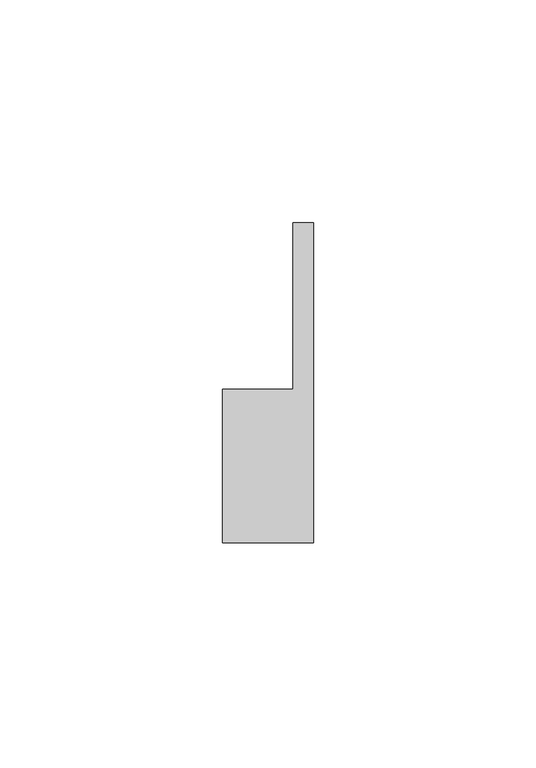
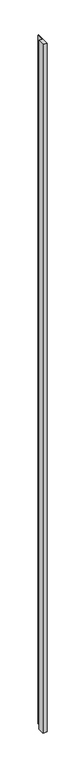
"""IFC4 building model written with IfcOpenShell, lengths in millimetres: proxy geometry, Generic Models 11:Generic Models 1:306267:Generic Models 1:306267 : Generic Models 11:Generic Models 1:306267:300405:Generic Models 1:306267:Generic Models 1:306267 : Generic Models 11:Generic Models 1:306267:300405 : Generic Models 11:Generic Models 1:306267:Generic Models 1:306267 : Generic Models 11:Generic Models 1:306267:300405:8 : Generic Models 11:Generic Models 1:306267:Generic Models 1:306267 : Generic Models 11:Generic Models 1:306267:300405:Generic Models 1:306267:Generic Models 1:306267 : Generic Models 11:Generic Models 1:306267:300405 : Generic Models 11:Generic Models 1:306267:Generic Models 1:306267 : Generic Models 11:Generic Models 1:306267:300405:300182."""

import ifcopenshell
import ifcopenshell.guid

model = None  # the IFC model being written
_history = None  # IfcOwnerHistory: only IFC2X3 demands one
_inside = {}  # id of a spatial element -> (the spatial element, [elements in it])
_under = {}  # id of a project, library or spatial element -> (it, [spatial elements below it])
_declared = {}  # id of a project -> (the project, [libraries it declares])
_typed = {}  # id of a type object -> (the type object, [elements of that type])
_made_of = {}  # id of a material, layer set ... -> (it, [elements and type objects made of it])


def new_model(schema):
    """Start an empty IFC model of exactly this schema.

    Asked for "IFC4X3", IfcOpenShell would pick the latest addendum, in which some entities
    have other attributes; the version numbers below select the first issue.
    IFC2X3 requires an IfcOwnerHistory on every rooted entity: one is made here for all.
    """
    global model, _history
    if schema == "IFC4X3":
        model = ifcopenshell.file(schema_version=(4, 3, 0, 0))
    else:
        model = ifcopenshell.file(schema=schema)
    _inside.clear()
    _under.clear()
    _declared.clear()
    _typed.clear()
    _made_of.clear()
    _history = None
    if model.schema == "IFC2X3":
        org = make("IfcOrganization", Name="unknown")
        user = make(
            "IfcPersonAndOrganization",
            ThePerson=make("IfcPerson", FamilyName="unknown"),
            TheOrganization=org,
        )
        app = make(
            "IfcApplication",
            ApplicationDeveloper=org,
            Version="unknown",
            ApplicationFullName="unknown",
            ApplicationIdentifier="unknown",
        )
        _history = make(
            "IfcOwnerHistory",
            OwningUser=user,
            OwningApplication=app,
            ChangeAction="ADDED",
            CreationDate=0,
        )
    return model


def make(cls, **values):
    """One entity of the class cls with the attributes given. An attribute that is None is left unset."""
    return model.create_entity(
        cls, **{name: value for name, value in values.items() if value is not None}
    )


def rooted(cls, **values):
    """An entity with a GlobalId (a new one), such as an element, a storey or a relation."""
    return make(cls, GlobalId=ifcopenshell.guid.new(), OwnerHistory=_history, **values)


def si_unit(unit_type, name, prefix=None):
    """IfcSIUnit, for example si_unit("LENGTHUNIT", "METRE", prefix="MILLI")."""
    return make("IfcSIUnit", UnitType=unit_type, Prefix=prefix, Name=name)


def assignment(units):
    """IfcUnitAssignment: the units of a project."""
    return None if units is None else make("IfcUnitAssignment", Units=units)


def point(xyz):
    """IfcCartesianPoint."""
    return None if xyz is None else make("IfcCartesianPoint", Coordinates=xyz)


def direction(xyz):
    """IfcDirection."""
    return None if xyz is None else make("IfcDirection", DirectionRatios=xyz)


def frame(location, z_axis=None, x_axis=None):
    """IfcAxis2Placement3D, a coordinate frame: its origin and axes. An axis left out is left unset."""
    return make(
        "IfcAxis2Placement3D",
        Location=point(location),
        Axis=direction(z_axis),
        RefDirection=direction(x_axis),
    )


def origin():
    """The frame at (0, 0, 0) with its axes left unset."""
    return frame((0.0, 0.0, 0.0))


def origin_with_axes():
    """The frame at (0, 0, 0) with the z axis (0, 0, 1) and the x axis (1, 0, 0) written out."""
    return frame((0.0, 0.0, 0.0), z_axis=(0.0, 0.0, 1.0), x_axis=(1.0, 0.0, 0.0))


def place(relative_to, where):
    """IfcLocalPlacement: puts the frame where relative to a parent placement (None: the world)."""
    return make(
        "IfcLocalPlacement", PlacementRelTo=relative_to, RelativePlacement=where
    )


def context(
    kind, dimensions, precision=None, world=None, true_north=None, identifier=None
):
    """IfcGeometricRepresentationContext, for example the 3D "Model" context."""
    return make(
        "IfcGeometricRepresentationContext",
        ContextIdentifier=identifier,
        ContextType=kind,
        CoordinateSpaceDimension=dimensions,
        Precision=precision,
        WorldCoordinateSystem=world,
        TrueNorth=true_north,
    )


def project(units=None, contexts=None):
    """IfcProject with its units and contexts."""
    return rooted(
        "IfcProject",
        Name="project",
        RepresentationContexts=contexts,
        UnitsInContext=assignment(units),
    )


def spatial(cls, under=None, at=None, **own):
    """A site, building, storey or space (cls), placed at a placement, below another one or the project."""
    s = rooted(cls, ObjectPlacement=at, **own)
    if under is not None:
        _under.setdefault(under.id(), (under, []))[1].append(s)
    return s


def polyline(points):
    """IfcPolyline through the points."""
    return make("IfcPolyline", Points=[point(p) for p in points])


def outline(outer, holes=None, kind="AREA"):
    """IfcArbitraryClosedProfileDef: a profile drawn as a closed curve; with holes, ...WithVoids."""
    if holes is None:
        return make("IfcArbitraryClosedProfileDef", ProfileType=kind, OuterCurve=outer)
    return make(
        "IfcArbitraryProfileDefWithVoids",
        ProfileType=kind,
        OuterCurve=outer,
        InnerCurves=holes,
    )


def extrude(swept, where, along, depth):
    """IfcExtrudedAreaSolid: the profile swept, set in the frame where, extruded along a direction by depth."""
    return make(
        "IfcExtrudedAreaSolid",
        SweptArea=swept,
        Position=where,
        ExtrudedDirection=direction(along),
        Depth=depth,
    )


def shape(context_of_items, identifier, shape_type, items):
    """IfcShapeRepresentation: the items that make up one representation, for example the "Body"."""
    return make(
        "IfcShapeRepresentation",
        ContextOfItems=context_of_items,
        RepresentationIdentifier=identifier,
        RepresentationType=shape_type,
        Items=items,
    )


def source(mapping_origin, context_of_items, identifier, shape_type, items):
    """IfcRepresentationMap: a shape defined once, which mapped items show again and again."""
    return make(
        "IfcRepresentationMap",
        MappingOrigin=mapping_origin,
        MappedRepresentation=shape(context_of_items, identifier, shape_type, items),
    )


def transform(
    local_origin,
    x_axis=None,
    y_axis=None,
    z_axis=None,
    scale=None,
    scale2=None,
    scale3=None,
    uniform=True,
):
    """IfcCartesianTransformationOperator3D, or its non-uniform kind. x_axis, y_axis, z_axis: its Axis1, 2, 3."""
    if uniform:
        return make(
            "IfcCartesianTransformationOperator3D",
            Axis1=direction(x_axis),
            Axis2=direction(y_axis),
            LocalOrigin=point(local_origin),
            Scale=scale,
            Axis3=direction(z_axis),
        )
    return make(
        "IfcCartesianTransformationOperator3DnonUniform",
        Axis1=direction(x_axis),
        Axis2=direction(y_axis),
        LocalOrigin=point(local_origin),
        Scale=scale,
        Axis3=direction(z_axis),
        Scale2=scale2,
        Scale3=scale3,
    )


def mapped(mapping_source, mapping_target):
    """IfcMappedItem: shows the shape of a source again, moved by a transform."""
    return make(
        "IfcMappedItem", MappingSource=mapping_source, MappingTarget=mapping_target
    )


def made_of(thing, what):
    """Note that an element or type object is made of a material, layer set ...; save() writes the relation."""
    if what is not None:
        _made_of.setdefault(what.id(), (what, []))[1].append(thing)
    return thing


def element(
    cls,
    number,
    at=None,
    inside=None,
    cuts=None,
    type_object=None,
    material=None,
    context=None,
    identifier="Body",
    shape_type=None,
    held_by="IfcProductDefinitionShape",
    body=None,
    shapes=None,
    **own,
):
    """One element of the class cls, such as IfcWall. Its Tag is "e" and its number.

    at: its placement. inside: the storey or other place that contains it. cuts: it is an
    opening in that element (IfcRelVoidsElement). A single representation is given by context,
    identifier, shape_type and body (its items); several are given by shapes. held_by: the class
    of the entity that holds the representations. save() writes the other relations.
    """
    e = rooted(cls, Tag="e%d" % number, ObjectPlacement=at, **own)
    if body is not None:
        shapes = [shape(context, identifier, shape_type, body)]
    if shapes is not None:
        e.Representation = make(held_by, Representations=shapes)
    if inside is not None:
        _inside.setdefault(inside.id(), (inside, []))[1].append(e)
    if cuts is not None:
        rooted(
            "IfcRelVoidsElement", RelatingBuildingElement=cuts, RelatedOpeningElement=e
        )
    if type_object is not None:
        _typed.setdefault(type_object.id(), (type_object, []))[1].append(e)
    return made_of(e, material)


def aggregate(whole, parts):
    """IfcRelAggregates: a whole, such as a stair, and the parts it consists of."""
    return rooted("IfcRelAggregates", RelatingObject=whole, RelatedObjects=parts)


def save(model, path):
    """Write the relations noted so far, then the file.

    IfcRelAggregates (storeys below a building ...), IfcRelContainedInSpatialStructure (elements
    in a storey), IfcRelDefinesByType, IfcRelAssociatesMaterial and IfcRelDeclares: one each for
    every whole, place, type object, material and project.
    """
    for whole, parts in _under.values():
        aggregate(whole, parts)
    for where, things in _inside.values():
        rooted(
            "IfcRelContainedInSpatialStructure",
            RelatedElements=things,
            RelatingStructure=where,
        )
    for kind, things in _typed.values():
        rooted("IfcRelDefinesByType", RelatedObjects=things, RelatingType=kind)
    for what, things in _made_of.values():
        rooted("IfcRelAssociatesMaterial", RelatedObjects=things, RelatingMaterial=what)
    for by, libraries in _declared.values():
        rooted("IfcRelDeclares", RelatingContext=by, RelatedDefinitions=libraries)
    model.write(path)


def generic_models_86148c45(model_context):
    return source(origin(), model_context, "Body", "SweptSolid", [
        extrude(outline(polyline([(570447.2188081, -579043.9402915), (570447.2188081, -579006.5153982), (570451.8591519, -579006.5153982), (570451.8591519, -579078.4496134), (570431.3487584, -579078.4496134), (570431.3487584, -579043.9402915), (570447.2188081, -579043.9402915)])), origin_with_axes(), (0.0, 0.0, 1.0), 3689.35),
    ])


if __name__ == "__main__":
    model = new_model("IFC4")
    model_context = context("Model", 3, world=origin())
    ifc_project = project(units=[si_unit("LENGTHUNIT", "METRE", prefix="MILLI")], contexts=[model_context])
    site = spatial("IfcSite", under=ifc_project)
    building = spatial("IfcBuilding", under=site)
    placement = place(None, origin())
    generic_models_shape = generic_models_86148c45(model_context)
    element("IfcBuildingElementProxy", 1, Name="Generic Models 11:Generic Models 1:306267:Generic Models 1:306267 : Generic Models 11:Generic Models 1:306267:300405:Generic Models 1:306267:Generic Models 1:306267 : Generic Models 11:Generic Models 1:306267:300405 : Generic Models 11:Generic Models 1:306267:Generic Models 1:306267 : Generic Models 11:Generic Models 1:306267:300405:8 : Generic Models 11:Generic Models 1:306267:Generic Models 1:306267 : Generic Models 11:Generic Models 1:306267:300405:Generic Models 1:306267:Generic Models 1:306267 : Generic Models 11:Generic Models 1:306267:300405 : Generic Models 11:Generic Models 1:306267:Generic Models 1:306267 : Generic Models 11:Generic Models 1:306267:300405:300182", ObjectType="Generic Models 11:Generic Models 1:306267:Generic Models 1:306267 : Generic Models 11:Generic Models 1:306267:300405:Generic Models 1:306267:Generic Models 1:306267 : Generic Models 11:Generic Models 1:306267:300405 : Generic Models 11:Generic Models 1:306267:Generic Models 1:306267 : Generic Models 11:Generic Models 1:306267:300405:8 : Generic Models 11:Generic Models 1:306267:Generic Models 1:306267 : Generic Models 11:Generic Models 1:306267:300405:Generic Models 1:306267:Generic Models 1:306267 : Generic Models 11:Generic Models 1:306267:300405 : Generic Models 11:Generic Models 1:306267:Generic Models 1:306267 : Generic Models 11:Generic Models 1:306267:300405:300182", at=placement, inside=building, context=model_context, shape_type="MappedRepresentation", body=[
        mapped(generic_models_shape, transform((0.0, 0.0, 0.0), x_axis=(1.0, 0.0, 0.0), y_axis=(0.0, 1.0, 0.0), z_axis=(0.0, 0.0, 1.0))),
    ])
    save(model, "model.ifc")

# Revit data of these elements
# Type "Generic Models 11:Generic Models 1:306267:Generic Models 1:306267 : Generic Models 11:Generic Models 1:306267:300405:Generic Models 1:306267:Generic Models 1:306267 : Generic Models 11:Generic Models 1:306267:300405 : Generic Models 11:Generic Models 1:306267:Generic Models 1:306267 : Generic Models 11:Generic Models 1:306267:300405:8 : Generic Models 11:Generic Models 1:306267:Generic Models 1:306267 : Generic Models 11:Generic Models 1:306267:300405:Generic Models 1:306267:Generic Models 1:306267 : Generic Models 11:Generic Models 1:306267:300405 : Generic Models 11:Generic Models 1:306267:Generic Models 1:306267 : Generic Models 11:Generic Models 1:306267:300405:300182"
#   NameOverride = "Generic Models 11:Generic Models 1:306267:Generic Models 1:306267 : Generic Models 11:Generic Models 1:306267:300405:Generic Models 1:306267:Generic Models 1:306267 : Generic Models 11:Generic Models 1:306267:300405 : Generic Models 11:Generic Models 1:306267:Generic Models 1:306267 : Generic Models 11:Generic Models 1:306267:300405:300182"
#   ObjectTypeOverride = "Generic Models 1:306267:Generic Models 1:306267 : Generic Models 11:Generic Models 1:306267:300405 : Generic Models 11:Generic Models 1:306267:Generic Models 1:306267 : Generic Models 11:Generic Models 1:306267:300405"
#   Reference = "Generic Models 1"
#   Tag = "300182"
# Element 1 (IfcBuildingElementProxy, "Generic Models 11:Generic Models 1:306267:Generic Models 1:306267 : Generic Models 11:Generic Models 1:306267:300405:Generic Models 1:306267:Generic Models 1:306267 : Generic Models 11:Generic Models 1:306267:300405 : Generic Models 11:Generic Models 1:306267:Generic Models 1:306267 : Generic Models 11:Generic Models 1:306267:300405:8 : Generic Models 11:Generic Models 1:306267:Generic Models 1:306267 : Generic Models 11:Generic Models 1:306267:300405:Generic Models 1:306267:Generic Models 1:306267 : Generic Models 11:Generic Models 1:306267:300405 : Generic Models 11:Generic Models 1:306267:Generic Models 1:306267 : Generic Models 11:Generic Models 1:306267:300405:300182")
#   Materials on its faces: "LOW VOLUMN EXPANDABLE FOAM INSULATION (CLASS A FLAME SPREAD)"
# Materials
#   "LOW VOLUMN EXPANDABLE FOAM INSULATION (CLASS A FLAME SPREAD)": class "Unassigned", colour RGB 213 216 95, transparency 0, Cost = 0
